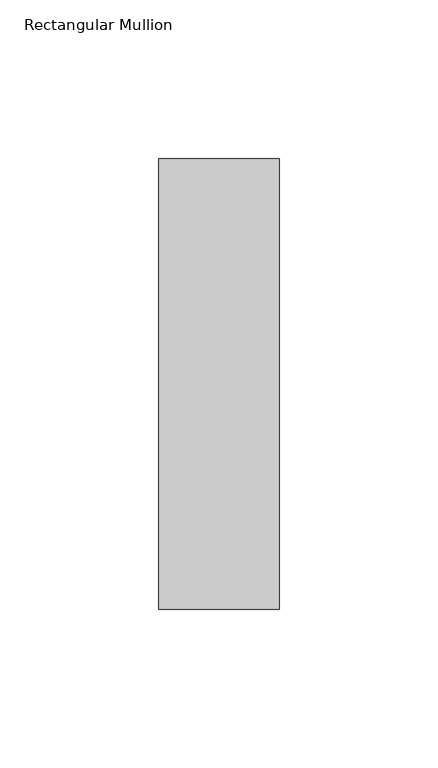
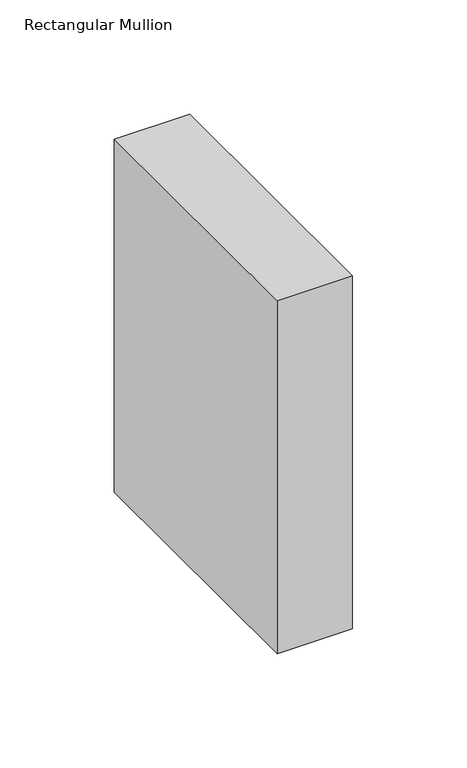
"""IFC4 building model written with IfcOpenShell, lengths in millimetres: member geometry, Rectangular Mullion : NLRS_21_CWM_hsb-regel 38x142_gen_rsf."""

from ifc_helpers import new_model, si_unit, frame, origin, place, context, project, spatial, polyline, outline, extrude, source, transform, mapped, element, save


def rectangular_mullion_6dedba73(model_context):
    return source(origin(), model_context, "Body", "SweptSolid", [
        extrude(outline(polyline([(0.0, -71.0), (-38.0, -71.0), (-38.0, 71.0), (0.0, 71.0), (0.0, -71.0)])), frame((0.0, 0.0, -187.9999997), z_axis=(0.0, 0.0, 1.0), x_axis=(1.0, 0.0, 0.0)), (0.0, 0.0, 1.0), 187.9999997),
    ])


if __name__ == "__main__":
    model = new_model("IFC4")
    model_context = context("Model", 3, world=origin())
    ifc_project = project(units=[si_unit("LENGTHUNIT", "METRE", prefix="MILLI")], contexts=[model_context])
    site = spatial("IfcSite", under=ifc_project)
    building = spatial("IfcBuilding", under=site)
    placement = place(None, origin())
    rectangular_mullion_shape = rectangular_mullion_6dedba73(model_context)
    element("IfcMember", 1, ObjectType="Rectangular Mullion : NLRS_21_CWM_hsb-regel 38x142_gen_rsf", at=placement, inside=building, context=model_context, shape_type="MappedRepresentation", body=[
        mapped(rectangular_mullion_shape, transform((0.0, 0.0, 0.0), x_axis=(1.0, 0.0, 0.0), y_axis=(0.0, 1.0, 0.0), z_axis=(0.0, 0.0, 1.0))),
    ])
    save(model, "model.ifc")

# Revit data of these elements
# Type "Rectangular Mullion : NLRS_21_CWM_hsb-regel 38x142_gen_rsf"
#   Export Type to IFC As = "IfcWall"
#   Type IfcGUID = "07M7mRoiH1CR8m_RSKIwpF"
#   Assembly Code = "21.10"
#   built-in parameter 1007322 = 0.465879 (stored number, unit not read)
#   built-in parameter 1007321 = 0.062336 (stored number, unit not read)
#   built-in parameter 1007320 = 0.062336 (stored number, unit not read)
# Element 1 (IfcMember, "Rectangular Mullion : NLRS_21_CWM_hsb-regel 38x142_gen_rsf")
#   Materials on its faces: "NLRS_i2_hout naaldhout vuren_gen_rsf"
# Materials
#   "NLRS_i2_hout naaldhout vuren_gen_rsf": class "I - Hout", colour RGB 234 199 147, transparency 0, Keynote = "i2", Manufacturer = "Revit Standards Foundation", URL = "www.revitstandards.org", Description = "hout vuren", Cost = 0
